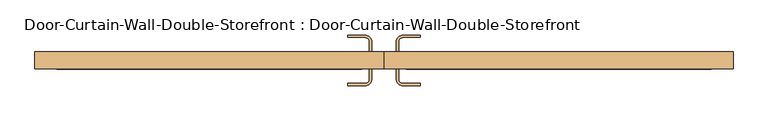
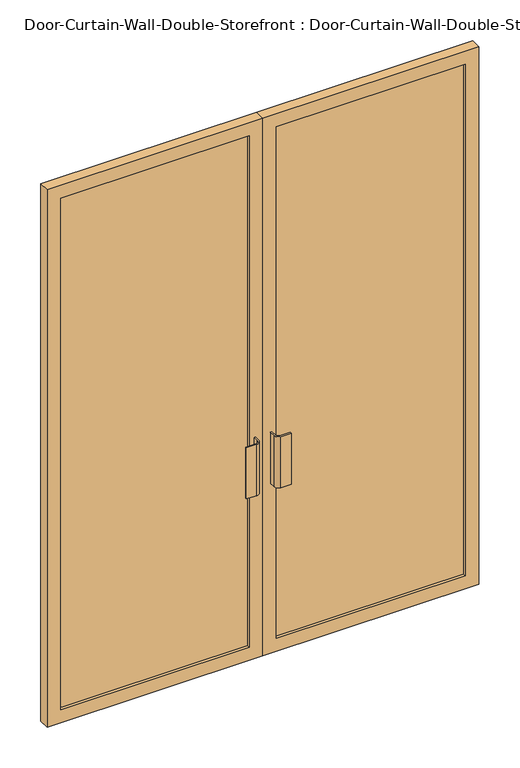
"""IFC4 building model written with IfcOpenShell, lengths in millimetres: door geometry, Door-Curtain-Wall-Double-Storefront : Door-Curtain-Wall-Double-Storefront."""

import ifcopenshell
import ifcopenshell.guid

model = None  # the IFC model being written
_history = None  # IfcOwnerHistory: only IFC2X3 demands one
_inside = {}  # id of a spatial element -> (the spatial element, [elements in it])
_under = {}  # id of a project, library or spatial element -> (it, [spatial elements below it])
_declared = {}  # id of a project -> (the project, [libraries it declares])
_typed = {}  # id of a type object -> (the type object, [elements of that type])
_made_of = {}  # id of a material, layer set ... -> (it, [elements and type objects made of it])


def new_model(schema):
    """Start an empty IFC model of exactly this schema.

    Asked for "IFC4X3", IfcOpenShell would pick the latest addendum, in which some entities
    have other attributes; the version numbers below select the first issue.
    IFC2X3 requires an IfcOwnerHistory on every rooted entity: one is made here for all.
    """
    global model, _history
    if schema == "IFC4X3":
        model = ifcopenshell.file(schema_version=(4, 3, 0, 0))
    else:
        model = ifcopenshell.file(schema=schema)
    _inside.clear()
    _under.clear()
    _declared.clear()
    _typed.clear()
    _made_of.clear()
    _history = None
    if model.schema == "IFC2X3":
        org = make("IfcOrganization", Name="unknown")
        user = make(
            "IfcPersonAndOrganization",
            ThePerson=make("IfcPerson", FamilyName="unknown"),
            TheOrganization=org,
        )
        app = make(
            "IfcApplication",
            ApplicationDeveloper=org,
            Version="unknown",
            ApplicationFullName="unknown",
            ApplicationIdentifier="unknown",
        )
        _history = make(
            "IfcOwnerHistory",
            OwningUser=user,
            OwningApplication=app,
            ChangeAction="ADDED",
            CreationDate=0,
        )
    return model


def make(cls, **values):
    """One entity of the class cls with the attributes given. An attribute that is None is left unset."""
    return model.create_entity(
        cls, **{name: value for name, value in values.items() if value is not None}
    )


def rooted(cls, **values):
    """An entity with a GlobalId (a new one), such as an element, a storey or a relation."""
    return make(cls, GlobalId=ifcopenshell.guid.new(), OwnerHistory=_history, **values)


def si_unit(unit_type, name, prefix=None):
    """IfcSIUnit, for example si_unit("LENGTHUNIT", "METRE", prefix="MILLI")."""
    return make("IfcSIUnit", UnitType=unit_type, Prefix=prefix, Name=name)


def assignment(units):
    """IfcUnitAssignment: the units of a project."""
    return None if units is None else make("IfcUnitAssignment", Units=units)


def point(xyz):
    """IfcCartesianPoint."""
    return None if xyz is None else make("IfcCartesianPoint", Coordinates=xyz)


def direction(xyz):
    """IfcDirection."""
    return None if xyz is None else make("IfcDirection", DirectionRatios=xyz)


def frame(location, z_axis=None, x_axis=None):
    """IfcAxis2Placement3D, a coordinate frame: its origin and axes. An axis left out is left unset."""
    return make(
        "IfcAxis2Placement3D",
        Location=point(location),
        Axis=direction(z_axis),
        RefDirection=direction(x_axis),
    )


def frame_2d(location, x_axis=None):
    """IfcAxis2Placement2D, a coordinate frame in the plane: its origin and x axis."""
    return make(
        "IfcAxis2Placement2D", Location=point(location), RefDirection=direction(x_axis)
    )


def origin():
    """The frame at (0, 0, 0) with its axes left unset."""
    return frame((0.0, 0.0, 0.0))


def place(relative_to, where):
    """IfcLocalPlacement: puts the frame where relative to a parent placement (None: the world)."""
    return make(
        "IfcLocalPlacement", PlacementRelTo=relative_to, RelativePlacement=where
    )


def context(
    kind, dimensions, precision=None, world=None, true_north=None, identifier=None
):
    """IfcGeometricRepresentationContext, for example the 3D "Model" context."""
    return make(
        "IfcGeometricRepresentationContext",
        ContextIdentifier=identifier,
        ContextType=kind,
        CoordinateSpaceDimension=dimensions,
        Precision=precision,
        WorldCoordinateSystem=world,
        TrueNorth=true_north,
    )


def project(units=None, contexts=None):
    """IfcProject with its units and contexts."""
    return rooted(
        "IfcProject",
        Name="project",
        RepresentationContexts=contexts,
        UnitsInContext=assignment(units),
    )


def spatial(cls, under=None, at=None, **own):
    """A site, building, storey or space (cls), placed at a placement, below another one or the project."""
    s = rooted(cls, ObjectPlacement=at, **own)
    if under is not None:
        _under.setdefault(under.id(), (under, []))[1].append(s)
    return s


def polyline(points):
    """IfcPolyline through the points."""
    return make("IfcPolyline", Points=[point(p) for p in points])


def circle_curve(where, radius):
    """IfcCircle in the frame where."""
    return make("IfcCircle", Position=where, Radius=radius)


def trimmed(basis, trim1, trim2, sense, master):
    """IfcTrimmedCurve: the piece of a basis curve between two trims."""
    return make(
        "IfcTrimmedCurve",
        BasisCurve=basis,
        Trim1=trim1,
        Trim2=trim2,
        SenseAgreement=sense,
        MasterRepresentation=master,
    )


def segment(curve, same_sense, transition):
    """IfcCompositeCurveSegment."""
    return make(
        "IfcCompositeCurveSegment",
        Transition=transition,
        SameSense=same_sense,
        ParentCurve=curve,
    )


def composite_curve(segments, self_intersect=None):
    """IfcCompositeCurve: segments joined end to end."""
    return make("IfcCompositeCurve", Segments=segments, SelfIntersect=self_intersect)


def outline(outer, holes=None, kind="AREA"):
    """IfcArbitraryClosedProfileDef: a profile drawn as a closed curve; with holes, ...WithVoids."""
    if holes is None:
        return make("IfcArbitraryClosedProfileDef", ProfileType=kind, OuterCurve=outer)
    return make(
        "IfcArbitraryProfileDefWithVoids",
        ProfileType=kind,
        OuterCurve=outer,
        InnerCurves=holes,
    )


def extrude(swept, where, along, depth):
    """IfcExtrudedAreaSolid: the profile swept, set in the frame where, extruded along a direction by depth."""
    return make(
        "IfcExtrudedAreaSolid",
        SweptArea=swept,
        Position=where,
        ExtrudedDirection=direction(along),
        Depth=depth,
    )


def shape(context_of_items, identifier, shape_type, items):
    """IfcShapeRepresentation: the items that make up one representation, for example the "Body"."""
    return make(
        "IfcShapeRepresentation",
        ContextOfItems=context_of_items,
        RepresentationIdentifier=identifier,
        RepresentationType=shape_type,
        Items=items,
    )


def source(mapping_origin, context_of_items, identifier, shape_type, items):
    """IfcRepresentationMap: a shape defined once, which mapped items show again and again."""
    return make(
        "IfcRepresentationMap",
        MappingOrigin=mapping_origin,
        MappedRepresentation=shape(context_of_items, identifier, shape_type, items),
    )


def transform(
    local_origin,
    x_axis=None,
    y_axis=None,
    z_axis=None,
    scale=None,
    scale2=None,
    scale3=None,
    uniform=True,
):
    """IfcCartesianTransformationOperator3D, or its non-uniform kind. x_axis, y_axis, z_axis: its Axis1, 2, 3."""
    if uniform:
        return make(
            "IfcCartesianTransformationOperator3D",
            Axis1=direction(x_axis),
            Axis2=direction(y_axis),
            LocalOrigin=point(local_origin),
            Scale=scale,
            Axis3=direction(z_axis),
        )
    return make(
        "IfcCartesianTransformationOperator3DnonUniform",
        Axis1=direction(x_axis),
        Axis2=direction(y_axis),
        LocalOrigin=point(local_origin),
        Scale=scale,
        Axis3=direction(z_axis),
        Scale2=scale2,
        Scale3=scale3,
    )


def mapped(mapping_source, mapping_target):
    """IfcMappedItem: shows the shape of a source again, moved by a transform."""
    return make(
        "IfcMappedItem", MappingSource=mapping_source, MappingTarget=mapping_target
    )


def made_of(thing, what):
    """Note that an element or type object is made of a material, layer set ...; save() writes the relation."""
    if what is not None:
        _made_of.setdefault(what.id(), (what, []))[1].append(thing)
    return thing


def element(
    cls,
    number,
    at=None,
    inside=None,
    cuts=None,
    type_object=None,
    material=None,
    context=None,
    identifier="Body",
    shape_type=None,
    held_by="IfcProductDefinitionShape",
    body=None,
    shapes=None,
    **own,
):
    """One element of the class cls, such as IfcWall. Its Tag is "e" and its number.

    at: its placement. inside: the storey or other place that contains it. cuts: it is an
    opening in that element (IfcRelVoidsElement). A single representation is given by context,
    identifier, shape_type and body (its items); several are given by shapes. held_by: the class
    of the entity that holds the representations. save() writes the other relations.
    """
    e = rooted(cls, Tag="e%d" % number, ObjectPlacement=at, **own)
    if body is not None:
        shapes = [shape(context, identifier, shape_type, body)]
    if shapes is not None:
        e.Representation = make(held_by, Representations=shapes)
    if inside is not None:
        _inside.setdefault(inside.id(), (inside, []))[1].append(e)
    if cuts is not None:
        rooted(
            "IfcRelVoidsElement", RelatingBuildingElement=cuts, RelatedOpeningElement=e
        )
    if type_object is not None:
        _typed.setdefault(type_object.id(), (type_object, []))[1].append(e)
    return made_of(e, material)


def aggregate(whole, parts):
    """IfcRelAggregates: a whole, such as a stair, and the parts it consists of."""
    return rooted("IfcRelAggregates", RelatingObject=whole, RelatedObjects=parts)


def save(model, path):
    """Write the relations noted so far, then the file.

    IfcRelAggregates (storeys below a building ...), IfcRelContainedInSpatialStructure (elements
    in a storey), IfcRelDefinesByType, IfcRelAssociatesMaterial and IfcRelDeclares: one each for
    every whole, place, type object, material and project.
    """
    for whole, parts in _under.values():
        aggregate(whole, parts)
    for where, things in _inside.values():
        rooted(
            "IfcRelContainedInSpatialStructure",
            RelatedElements=things,
            RelatingStructure=where,
        )
    for kind, things in _typed.values():
        rooted("IfcRelDefinesByType", RelatedObjects=things, RelatingType=kind)
    for what, things in _made_of.values():
        rooted("IfcRelAssociatesMaterial", RelatedObjects=things, RelatingMaterial=what)
    for by, libraries in _declared.values():
        rooted("IfcRelDeclares", RelatingContext=by, RelatedDefinitions=libraries)
    model.write(path)


def door_curtain_wall_double_storefront_door_curtain_wall_double_b989ae86(model_context):
    return source(origin(), model_context, "Body", "SweptSolid", [
        extrude(outline(polyline([(2406.65, 0.7668501), (0.0, 0.7668501), (0.0, 914.4), (2406.65, 914.4), (2406.65, 0.7668501)]), holes=[polyline([(2349.5, 57.9168501), (2349.5, 857.25), (57.15, 857.25), (57.15, 57.9168501), (2349.5, 57.9168501)])]), frame((0.0, -57.15, 0.0), z_axis=(0.0, 1.0, 0.0), x_axis=(0.0, 0.0, 1.0)), (0.0, 0.0, 1.0), 44.45),
        extrude(outline(polyline([(2406.65, -0.8206499), (2406.65, -914.4), (0.0, -914.4), (0.0, -0.8206499), (2406.65, -0.8206499)]), holes=[polyline([(2349.5, -857.25), (2349.5, -57.9706499), (57.15, -57.9706499), (57.15, -857.25), (2349.5, -857.25)])]), frame((0.0, -57.15, 0.0), z_axis=(0.0, 1.0, 0.0), x_axis=(0.0, 0.0, 1.0)), (0.0, 0.0, 1.0), 44.45),
        extrude(outline(polyline([(857.25, -25.4), (857.25, -44.45), (57.9168501, -44.45), (57.9168501, -25.4), (857.25, -25.4)])), frame((0.0, 0.0, 57.15), z_axis=(0.0, 0.0, 1.0), x_axis=(1.0, 0.0, 0.0)), (0.0, 0.0, 1.0), 2292.35),
        extrude(outline(polyline([(-57.9706499, -25.4), (-57.9706499, -44.45), (-857.25, -44.45), (-857.25, -25.4), (-57.9706499, -25.4)])), frame((0.0, 0.0, 57.15), z_axis=(0.0, 0.0, 1.0), x_axis=(1.0, 0.0, 0.0)), (0.0, 0.0, 1.0), 2292.35),
        extrude(outline(composite_curve([segment(polyline([(-31.7768999, 12.7), (-31.7768999, -12.7), (-38.1268999, -12.7), (-38.1268999, 12.7)]), True, "CONTINUOUS"), segment(trimmed(circle_curve(frame_2d((-50.8268999, 12.7)), 12.7), [point((-38.1268999, 12.7))], [point((-50.8268999, 25.4))], True, "CARTESIAN"), True, "CONTINUOUS"), segment(polyline([(-50.8268999, 25.4), (-95.2768999, 25.4), (-95.2768999, 31.75), (-50.8268999, 31.75)]), True, "CONTINUOUS"), segment(trimmed(circle_curve(frame_2d((-50.8268999, 12.7)), 19.05), [point((-50.8268999, 31.75))], [point((-31.7768999, 12.7))], False, "CARTESIAN"), True, "CONTINUOUS")], self_intersect=False)), frame((0.0, 0.0, 762.0), z_axis=(0.0, 0.0, 1.0), x_axis=(1.0, 0.0, 0.0)), (0.0, 0.0, 1.0), 228.6),
        extrude(outline(composite_curve([segment(trimmed(circle_curve(frame_2d((50.7731001, 12.7)), 19.05), [point((31.7231001, 12.7))], [point((50.7731001, 31.75))], False, "CARTESIAN"), True, "CONTINUOUS"), segment(polyline([(50.7731001, 31.75), (95.2231001, 31.75), (95.2231001, 25.4), (50.7731001, 25.4)]), True, "CONTINUOUS"), segment(trimmed(circle_curve(frame_2d((50.7731001, 12.7)), 12.7), [point((50.7731001, 25.4))], [point((38.0731001, 12.7))], True, "CARTESIAN"), True, "CONTINUOUS"), segment(polyline([(38.0731001, 12.7), (38.0731001, -12.7), (31.7231001, -12.7), (31.7231001, 12.7)]), True, "CONTINUOUS")], self_intersect=False)), frame((0.0, 0.0, 762.0), z_axis=(0.0, 0.0, 1.0), x_axis=(1.0, 0.0, 0.0)), (0.0, 0.0, 1.0), 228.6),
        extrude(outline(composite_curve([segment(trimmed(circle_curve(frame_2d((-50.8268999, -82.55)), 19.05), [point((-31.7768999, -82.55))], [point((-50.8268999, -101.6))], False, "CARTESIAN"), True, "CONTINUOUS"), segment(polyline([(-50.8268999, -101.6), (-95.2768999, -101.6), (-95.2768999, -95.25), (-50.8268999, -95.25)]), True, "CONTINUOUS"), segment(trimmed(circle_curve(frame_2d((-50.8268999, -82.55)), 12.7), [point((-50.8268999, -95.25))], [point((-38.1268999, -82.55))], True, "CARTESIAN"), True, "CONTINUOUS"), segment(polyline([(-38.1268999, -82.55), (-38.1268999, -57.15), (-31.7768999, -57.15), (-31.7768999, -82.55)]), True, "CONTINUOUS")], self_intersect=False)), frame((0.0, 0.0, 762.0), z_axis=(0.0, 0.0, 1.0), x_axis=(1.0, 0.0, 0.0)), (0.0, 0.0, 1.0), 228.6),
        extrude(outline(composite_curve([segment(polyline([(31.7231001, -82.55), (31.7231001, -57.15), (38.0731001, -57.15), (38.0731001, -82.55)]), True, "CONTINUOUS"), segment(trimmed(circle_curve(frame_2d((50.7731001, -82.55)), 12.7), [point((38.0731001, -82.55))], [point((50.7731001, -95.25))], True, "CARTESIAN"), True, "CONTINUOUS"), segment(polyline([(50.7731001, -95.25), (95.2231001, -95.25), (95.2231001, -101.6), (50.7731001, -101.6)]), True, "CONTINUOUS"), segment(trimmed(circle_curve(frame_2d((50.7731001, -82.55)), 19.05), [point((50.7731001, -101.6))], [point((31.7231001, -82.55))], False, "CARTESIAN"), True, "CONTINUOUS")], self_intersect=False)), frame((0.0, 0.0, 762.0), z_axis=(0.0, 0.0, 1.0), x_axis=(1.0, 0.0, 0.0)), (0.0, 0.0, 1.0), 228.6),
    ])


if __name__ == "__main__":
    model = new_model("IFC4")
    model_context = context("Model", 3, world=origin())
    ifc_project = project(units=[si_unit("LENGTHUNIT", "METRE", prefix="MILLI")], contexts=[model_context])
    site = spatial("IfcSite", under=ifc_project)
    building = spatial("IfcBuilding", under=site)
    placement = place(None, origin())
    door_curtain_wall_double_storefront_door_curtain_wall_double_shape = door_curtain_wall_double_storefront_door_curtain_wall_double_b989ae86(model_context)
    element("IfcDoor", 1, ObjectType="Door-Curtain-Wall-Double-Storefront : Door-Curtain-Wall-Double-Storefront", at=placement, inside=building, context=model_context, shape_type="MappedRepresentation", body=[
        mapped(door_curtain_wall_double_storefront_door_curtain_wall_double_shape, transform((0.0, 0.0, 0.0), x_axis=(1.0, 0.0, 0.0), y_axis=(0.0, 1.0, 0.0), z_axis=(0.0, 0.0, 1.0))),
    ])
    save(model, "model.ifc")

# Revit data of these elements
# Type "Door-Curtain-Wall-Double-Storefront : Door-Curtain-Wall-Double-Storefront"
#   Type Mark = "15"
#   Fire Rating = "--"
#   Construction Type Id = "opn-d46"
#   Assembly Code = "B2030100"
#   Analytic Construction = "Metal frame, double glass door"
#   Thickness = 0' - 1 3/4"
#   Width [instance default] = 6' - 0"
#   Thermal Resistance (R) = 1.3794 (h·ft²·°F)/BTU
#   Swing Angle [instance default] = 90.00°
#   Panel Width [instance default] = 3' - 0"
#   Offset = 0' - 2 1/4"
#   Heat Transfer Coefficient (U) = 0.7250 BTU/(h·ft²·°F)
#   Define Thermal Properties by = 1
#   Function = 1
#   Frame Material = Aluminum
#   Door Handle Material = Aluminum
#   Glazing = Glass
#   Visual Light Transmittance = 0
#   Solar Heat Gain Coefficient = 0
# Element 1 (IfcDoor, "Door-Curtain-Wall-Double-Storefront : Door-Curtain-Wall-Double-Storefront")
#   Materials on its faces: "Aluminum", "Glass"
# Materials
#   "Aluminum": class "Metal", colour RGB 247 247 247, transparency 0, Description = "Aluminum 6061", Cost = 0
#   "Glass": class "Glass", colour RGB 0 0 255, transparency 0.75, Description = "Soda Lime Glass", Cost = 0
